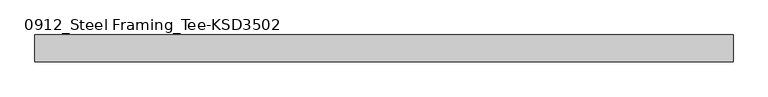
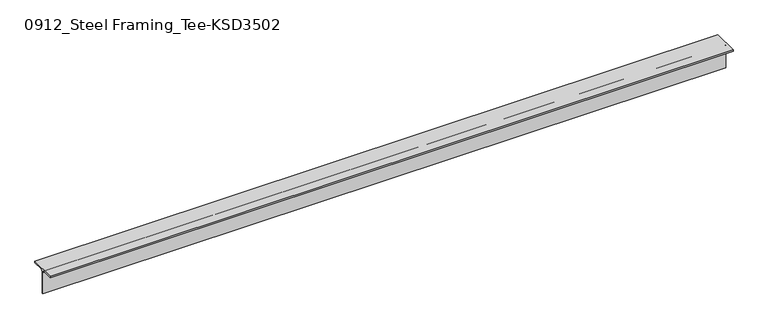
"""IFC4 building model written with IfcOpenShell, lengths in millimetres: member geometry, 0912_Steel Framing_Tee-KSD3502 : H_SB_ASB_CT-150x150x6.5x9."""

from ifc_helpers import new_model, si_unit, point, frame, frame_2d, origin, place, context, project, spatial, polyline, circle_curve, trimmed, segment, composite_curve, outline, extrude, source, transform, mapped, element, save


def member_0912_steel_framing_tee_ksd3502_42f31cb5(model_context):
    return source(origin(), model_context, "Body", "SweptSolid", [
        extrude(outline(composite_curve([segment(polyline([(-75.0, 75.0), (75.0, 75.0), (75.0, 66.0), (16.25, 66.0)]), True, "CONTINUOUS"), segment(trimmed(circle_curve(frame_2d((16.25, 53.0)), 13.0), [point((16.25, 66.0))], [point((3.25, 53.0))], True, "CARTESIAN"), True, "CONTINUOUS"), segment(polyline([(3.25, 53.0), (3.25, -75.0), (-3.25, -75.0), (-3.25, 53.0)]), True, "CONTINUOUS"), segment(trimmed(circle_curve(frame_2d((-16.25, 53.0)), 13.0), [point((-3.25, 53.0))], [point((-16.25, 66.0))], True, "CARTESIAN"), True, "CONTINUOUS"), segment(polyline([(-16.25, 66.0), (-75.0, 66.0), (-75.0, 75.0)]), True, "CONTINUOUS")], self_intersect=False)), frame((-1932.85, 0.0, 0.0), z_axis=(1.0, 0.0, 0.0), x_axis=(0.0, 1.0, 0.0)), (0.0, 0.0, 1.0), 3898.3),
    ])


if __name__ == "__main__":
    model = new_model("IFC4")
    model_context = context("Model", 3, world=origin())
    ifc_project = project(units=[si_unit("LENGTHUNIT", "METRE", prefix="MILLI")], contexts=[model_context])
    site = spatial("IfcSite", under=ifc_project)
    building = spatial("IfcBuilding", under=site)
    placement = place(None, origin())
    member_0912_steel_framing_tee_ksd3502_shape = member_0912_steel_framing_tee_ksd3502_42f31cb5(model_context)
    element("IfcMember", 1, ObjectType="0912_Steel Framing_Tee-KSD3502 : H_SB_ASB_CT-150x150x6.5x9", at=placement, inside=building, context=model_context, shape_type="MappedRepresentation", body=[
        mapped(member_0912_steel_framing_tee_ksd3502_shape, transform((0.0, 0.0, 0.0), x_axis=(1.0, 0.0, 0.0), y_axis=(0.0, 1.0, 0.0), z_axis=(0.0, 0.0, 1.0))),
    ])
    save(model, "model.ifc")

# Revit data of these elements
# Type "0912_Steel Framing_Tee-KSD3502 : H_SB_ASB_CT-150x150x6.5x9"
#   H_WM Code_1 = "S01AA003-00001 | Main Steel Structure Fabrication Work | Shelter/Building | Light Steel - Standard (30KG/M>Weight) | Material: (   )"
#   H_WM Code_2 = "S03AA029-00001 | Main Steel Structure Erection Work | Shelter/Building | Light Steel (30KG/M>Weight) | Material: (   )"
#   H_WM Code_3 = "S01AA010-00001 | Main Steel Structure Fabrication Work | Shelter/Building | Steel Painting/Coating | for Non-Fireproofed Steel Surface, Surface Preparation, Primer, Second & Final Coat | Material: (   )"
#   H_Q'ty Cal Type Tag = "SB-Q2"
#   Width = 15.0 cm
#   Web Thickness = 0.65 cm
#   Web Fillet = 1.3 cm
#   Section Area = 23.39 cm²
#   Perimeter = 0.60 m²/m
#   Nominal Weight = 18.40 kgf/m
#   Height = 15.0 cm
#   Flange Thickness = 0.9 cm
#   Centroid Vertical = 7.5 cm
#   Centroid Horizontal = 7.5 cm
#   Length [instance default] = 1.5000 m
#   Structural Material [instance default] = Steel, 45-345
#   Warping Constant = (empty or 0)
#   Torsional Moment of Inertia = 0
#   Section Name Key = ""
#   Plastic Modulus weak axis = 0
#   Plastic Modulus strong axis = 0
#   Moment of Inertia weak axis = 0
#   Moment of Inertia strong axis = 0
#   Elastic Modulus weak axis = 0
#   Elastic Modulus strong axis = 0
#   Bolt Spacing = 0
#   Assembly Code = ""
# Element 1 (IfcMember, "0912_Steel Framing_Tee-KSD3502 : H_SB_ASB_CT-150x150x6.5x9")
#   Structural Material = none
# Materials
#   "Steel, 45-345": class "Metal", colour RGB 189 187 185, transparency 0, Description = "Steel 345 MPa", Cost = 0
